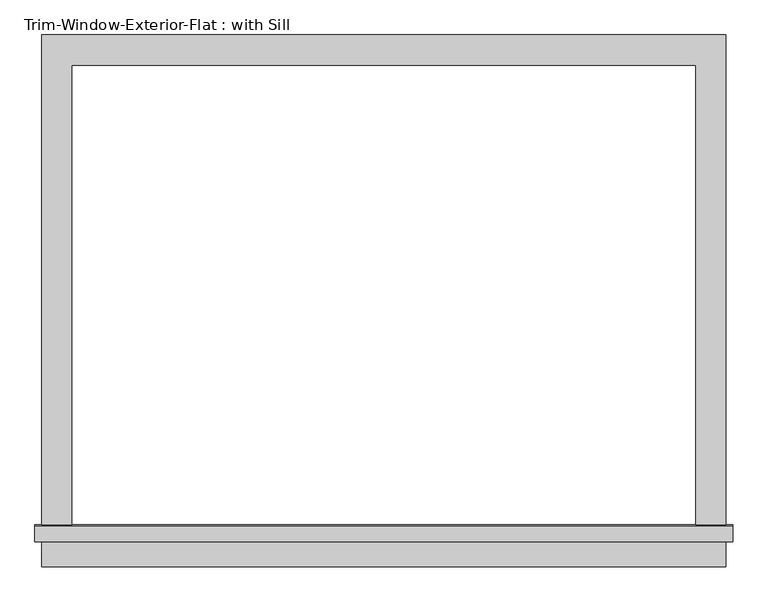
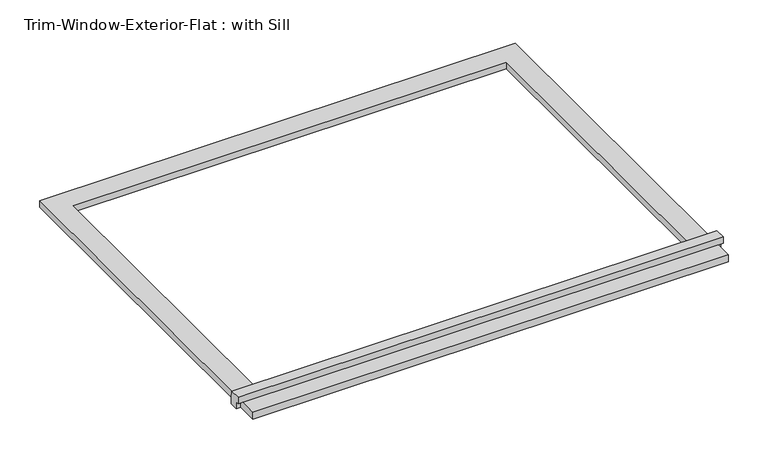
"""IFC4 building model written with IfcOpenShell, lengths in millimetres: proxy geometry, Trim-Window-Exterior-Flat : with Sill."""

from ifc_helpers import new_model, si_unit, frame, origin, origin_with_axes, place, context, project, spatial, polyline, outline, extrude, source, transform, mapped, element, save


def trim_window_exterior_flat_with_sill_a6ca139b(model_context):
    return source(origin(), model_context, "Body", "SweptSolid", [
        extrude(outline(polyline([(647.7, -892.1323709), (647.7, -949.2823709), (-647.7, -949.2823709), (-647.7, -892.1323709), (647.7, -892.1323709)])), origin_with_axes(), (0.0, 0.0, 1.0), 19.05),
        extrude(outline(polyline([(-901.7, 38.1), (-872.4080645, 38.1), (-869.95, 19.05), (-869.95, 0.0), (-892.1323709, 0.0), (-892.1323709, 19.05), (-901.7, 19.05), (-901.7, 38.1)])), frame((-660.4, 0.0, 0.0), z_axis=(1.0, 0.0, 0.0), x_axis=(0.0, 1.0, 0.0)), (0.0, 0.0, 1.0), 1320.8),
        extrude(outline(polyline([(-647.7, 57.15), (647.7, 57.15), (647.7, -869.95), (590.55, -869.95), (590.55, 0.0), (-590.55, 0.0), (-590.55, -869.95), (-647.7, -869.95), (-647.7, 57.15)])), origin_with_axes(), (0.0, 0.0, 1.0), 19.05),
    ])


if __name__ == "__main__":
    model = new_model("IFC4")
    model_context = context("Model", 3, world=origin())
    ifc_project = project(units=[si_unit("LENGTHUNIT", "METRE", prefix="MILLI")], contexts=[model_context])
    site = spatial("IfcSite", under=ifc_project)
    building = spatial("IfcBuilding", under=site)
    placement = place(None, origin())
    trim_window_exterior_flat_with_sill_shape = trim_window_exterior_flat_with_sill_a6ca139b(model_context)
    element("IfcBuildingElementProxy", 1, Name="Trim-Window-Exterior-Flat : with Sill", ObjectType="Trim-Window-Exterior-Flat : with Sill", at=placement, inside=building, context=model_context, shape_type="MappedRepresentation", body=[
        mapped(trim_window_exterior_flat_with_sill_shape, transform((0.0, 0.0, 0.0), x_axis=(1.0, 0.0, 0.0), y_axis=(0.0, 1.0, 0.0), z_axis=(0.0, 0.0, 1.0))),
    ])
    save(model, "model.ifc")

# Revit data of these elements
# Type "Trim-Window-Exterior-Flat : with Sill"
#   Trim Width = 0' - 2 1/4"
#   Trim Thickness_Picture Frame = 0' - 1 1/4"
#   Trim Thickness_with Sill = 0' - 0 3/4"
#   Sill Thickness = 0' - 1 1/4"
#   Opening Width [instance default] = 2' - 0"
#   Opening Height [instance default] = 3' - 0"
#   Default Elevation = 4' - 0"
#   Sill = yes
#   Picture Frame = no
#   Trim Material [instance default] = none
# Element 1 (IfcBuildingElementProxy, "Trim-Window-Exterior-Flat : with Sill")
#   Opening Width = 3' - 10 1/2"
#   Opening Height = 2' - 10 1/4"
#   Trim Material = Clad - White
#   Materials on its faces: "Clad - White"
# Materials
#   "Clad - White": class "Wood", colour RGB 242 242 238, transparency 0, Cost = 0
